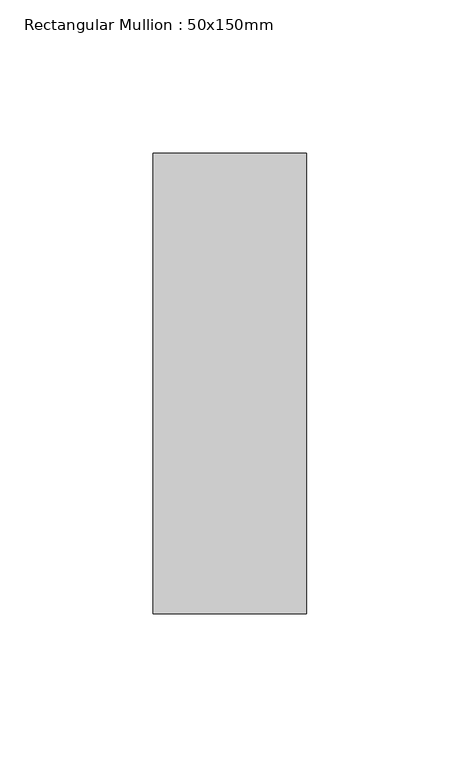
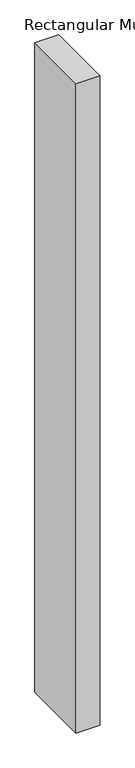
"""IFC4 building model written with IfcOpenShell, lengths in millimetres: member geometry, Rectangular Mullion : 50x150mm."""

from ifc_helpers import new_model, si_unit, frame, origin, place, context, project, spatial, polyline, outline, extrude, source, transform, mapped, element, save


def rectangular_mullion_50x150mm_f6f7edf2(model_context):
    return source(origin(), model_context, "Body", "SweptSolid", [
        extrude(outline(polyline([(25.0, 75.0), (25.0, -75.0), (-25.0, -75.0), (-25.0, 75.0), (25.0, 75.0)])), frame((0.0, 0.0, -1449.9999998), z_axis=(0.0, 0.0, 1.0), x_axis=(1.0, 0.0, 0.0)), (0.0, 0.0, 1.0), 1449.9999998),
    ])


if __name__ == "__main__":
    model = new_model("IFC4")
    model_context = context("Model", 3, world=origin())
    ifc_project = project(units=[si_unit("LENGTHUNIT", "METRE", prefix="MILLI")], contexts=[model_context])
    site = spatial("IfcSite", under=ifc_project)
    building = spatial("IfcBuilding", under=site)
    placement = place(None, origin())
    rectangular_mullion_50x150mm_shape = rectangular_mullion_50x150mm_f6f7edf2(model_context)
    element("IfcMember", 1, ObjectType="Rectangular Mullion : 50x150mm", at=placement, inside=building, context=model_context, shape_type="MappedRepresentation", body=[
        mapped(rectangular_mullion_50x150mm_shape, transform((0.0, 0.0, 0.0), x_axis=(1.0, 0.0, 0.0), y_axis=(0.0, 1.0, 0.0), z_axis=(0.0, 0.0, 1.0))),
    ])
    save(model, "model.ifc")

# Revit data of these elements
# Type "Rectangular Mullion : 50x150mm"
#   Keynote = "H11"
#   built-in parameter 1007304 = 0.492126 (stored number, unit not read)
#   built-in parameter 1007301 = 0.082021 (stored number, unit not read)
#   built-in parameter 1007300 = 0.082021 (stored number, unit not read)
# Element 1 (IfcMember, "Rectangular Mullion : 50x150mm")
#   Materials on its faces: "Aluminium"
# Materials
#   "Aluminium": class "Metal", colour RGB 247 247 247, transparency 0, Description = "Aluminium 6061", Cost = 0
